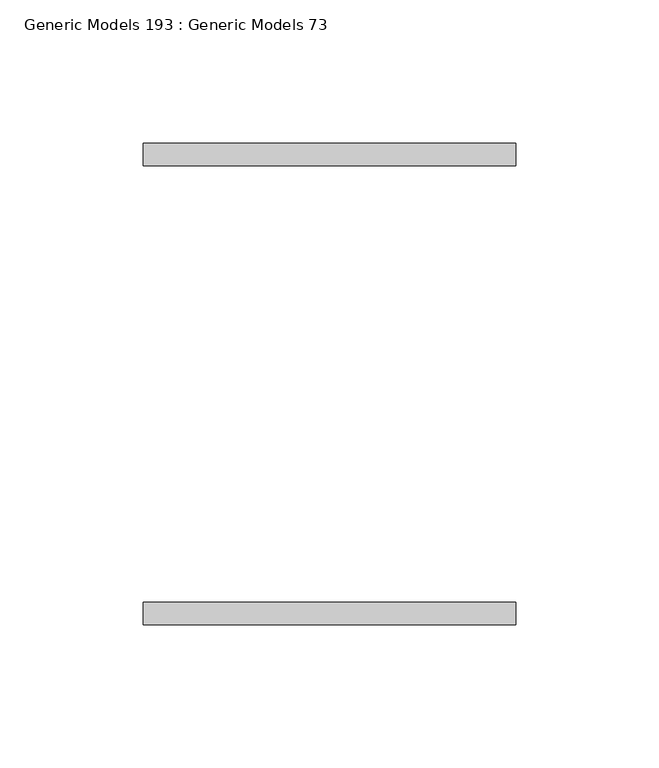
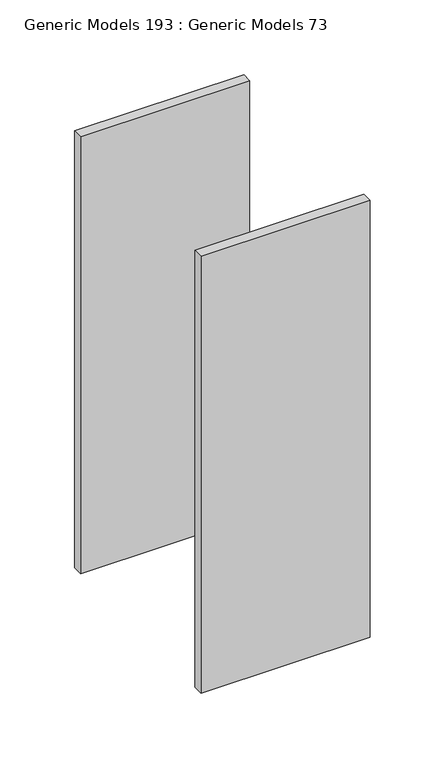
"""IFC4 building model written with IfcOpenShell, lengths in millimetres: proxy geometry, Generic Models 193 : Generic Models 73."""

import ifcopenshell
import ifcopenshell.guid

model = None  # the IFC model being written
_history = None  # IfcOwnerHistory: only IFC2X3 demands one
_inside = {}  # id of a spatial element -> (the spatial element, [elements in it])
_under = {}  # id of a project, library or spatial element -> (it, [spatial elements below it])
_declared = {}  # id of a project -> (the project, [libraries it declares])
_typed = {}  # id of a type object -> (the type object, [elements of that type])
_made_of = {}  # id of a material, layer set ... -> (it, [elements and type objects made of it])


def new_model(schema):
    """Start an empty IFC model of exactly this schema.

    Asked for "IFC4X3", IfcOpenShell would pick the latest addendum, in which some entities
    have other attributes; the version numbers below select the first issue.
    IFC2X3 requires an IfcOwnerHistory on every rooted entity: one is made here for all.
    """
    global model, _history
    if schema == "IFC4X3":
        model = ifcopenshell.file(schema_version=(4, 3, 0, 0))
    else:
        model = ifcopenshell.file(schema=schema)
    _inside.clear()
    _under.clear()
    _declared.clear()
    _typed.clear()
    _made_of.clear()
    _history = None
    if model.schema == "IFC2X3":
        org = make("IfcOrganization", Name="unknown")
        user = make(
            "IfcPersonAndOrganization",
            ThePerson=make("IfcPerson", FamilyName="unknown"),
            TheOrganization=org,
        )
        app = make(
            "IfcApplication",
            ApplicationDeveloper=org,
            Version="unknown",
            ApplicationFullName="unknown",
            ApplicationIdentifier="unknown",
        )
        _history = make(
            "IfcOwnerHistory",
            OwningUser=user,
            OwningApplication=app,
            ChangeAction="ADDED",
            CreationDate=0,
        )
    return model


def make(cls, **values):
    """One entity of the class cls with the attributes given. An attribute that is None is left unset."""
    return model.create_entity(
        cls, **{name: value for name, value in values.items() if value is not None}
    )


def rooted(cls, **values):
    """An entity with a GlobalId (a new one), such as an element, a storey or a relation."""
    return make(cls, GlobalId=ifcopenshell.guid.new(), OwnerHistory=_history, **values)


def si_unit(unit_type, name, prefix=None):
    """IfcSIUnit, for example si_unit("LENGTHUNIT", "METRE", prefix="MILLI")."""
    return make("IfcSIUnit", UnitType=unit_type, Prefix=prefix, Name=name)


def assignment(units):
    """IfcUnitAssignment: the units of a project."""
    return None if units is None else make("IfcUnitAssignment", Units=units)


def point(xyz):
    """IfcCartesianPoint."""
    return None if xyz is None else make("IfcCartesianPoint", Coordinates=xyz)


def direction(xyz):
    """IfcDirection."""
    return None if xyz is None else make("IfcDirection", DirectionRatios=xyz)


def frame(location, z_axis=None, x_axis=None):
    """IfcAxis2Placement3D, a coordinate frame: its origin and axes. An axis left out is left unset."""
    return make(
        "IfcAxis2Placement3D",
        Location=point(location),
        Axis=direction(z_axis),
        RefDirection=direction(x_axis),
    )


def origin():
    """The frame at (0, 0, 0) with its axes left unset."""
    return frame((0.0, 0.0, 0.0))


def place(relative_to, where):
    """IfcLocalPlacement: puts the frame where relative to a parent placement (None: the world)."""
    return make(
        "IfcLocalPlacement", PlacementRelTo=relative_to, RelativePlacement=where
    )


def context(
    kind, dimensions, precision=None, world=None, true_north=None, identifier=None
):
    """IfcGeometricRepresentationContext, for example the 3D "Model" context."""
    return make(
        "IfcGeometricRepresentationContext",
        ContextIdentifier=identifier,
        ContextType=kind,
        CoordinateSpaceDimension=dimensions,
        Precision=precision,
        WorldCoordinateSystem=world,
        TrueNorth=true_north,
    )


def project(units=None, contexts=None):
    """IfcProject with its units and contexts."""
    return rooted(
        "IfcProject",
        Name="project",
        RepresentationContexts=contexts,
        UnitsInContext=assignment(units),
    )


def spatial(cls, under=None, at=None, **own):
    """A site, building, storey or space (cls), placed at a placement, below another one or the project."""
    s = rooted(cls, ObjectPlacement=at, **own)
    if under is not None:
        _under.setdefault(under.id(), (under, []))[1].append(s)
    return s


def polyline(points):
    """IfcPolyline through the points."""
    return make("IfcPolyline", Points=[point(p) for p in points])


def outline(outer, holes=None, kind="AREA"):
    """IfcArbitraryClosedProfileDef: a profile drawn as a closed curve; with holes, ...WithVoids."""
    if holes is None:
        return make("IfcArbitraryClosedProfileDef", ProfileType=kind, OuterCurve=outer)
    return make(
        "IfcArbitraryProfileDefWithVoids",
        ProfileType=kind,
        OuterCurve=outer,
        InnerCurves=holes,
    )


def extrude(swept, where, along, depth):
    """IfcExtrudedAreaSolid: the profile swept, set in the frame where, extruded along a direction by depth."""
    return make(
        "IfcExtrudedAreaSolid",
        SweptArea=swept,
        Position=where,
        ExtrudedDirection=direction(along),
        Depth=depth,
    )


def shape(context_of_items, identifier, shape_type, items):
    """IfcShapeRepresentation: the items that make up one representation, for example the "Body"."""
    return make(
        "IfcShapeRepresentation",
        ContextOfItems=context_of_items,
        RepresentationIdentifier=identifier,
        RepresentationType=shape_type,
        Items=items,
    )


def source(mapping_origin, context_of_items, identifier, shape_type, items):
    """IfcRepresentationMap: a shape defined once, which mapped items show again and again."""
    return make(
        "IfcRepresentationMap",
        MappingOrigin=mapping_origin,
        MappedRepresentation=shape(context_of_items, identifier, shape_type, items),
    )


def transform(
    local_origin,
    x_axis=None,
    y_axis=None,
    z_axis=None,
    scale=None,
    scale2=None,
    scale3=None,
    uniform=True,
):
    """IfcCartesianTransformationOperator3D, or its non-uniform kind. x_axis, y_axis, z_axis: its Axis1, 2, 3."""
    if uniform:
        return make(
            "IfcCartesianTransformationOperator3D",
            Axis1=direction(x_axis),
            Axis2=direction(y_axis),
            LocalOrigin=point(local_origin),
            Scale=scale,
            Axis3=direction(z_axis),
        )
    return make(
        "IfcCartesianTransformationOperator3DnonUniform",
        Axis1=direction(x_axis),
        Axis2=direction(y_axis),
        LocalOrigin=point(local_origin),
        Scale=scale,
        Axis3=direction(z_axis),
        Scale2=scale2,
        Scale3=scale3,
    )


def mapped(mapping_source, mapping_target):
    """IfcMappedItem: shows the shape of a source again, moved by a transform."""
    return make(
        "IfcMappedItem", MappingSource=mapping_source, MappingTarget=mapping_target
    )


def made_of(thing, what):
    """Note that an element or type object is made of a material, layer set ...; save() writes the relation."""
    if what is not None:
        _made_of.setdefault(what.id(), (what, []))[1].append(thing)
    return thing


def element(
    cls,
    number,
    at=None,
    inside=None,
    cuts=None,
    type_object=None,
    material=None,
    context=None,
    identifier="Body",
    shape_type=None,
    held_by="IfcProductDefinitionShape",
    body=None,
    shapes=None,
    **own,
):
    """One element of the class cls, such as IfcWall. Its Tag is "e" and its number.

    at: its placement. inside: the storey or other place that contains it. cuts: it is an
    opening in that element (IfcRelVoidsElement). A single representation is given by context,
    identifier, shape_type and body (its items); several are given by shapes. held_by: the class
    of the entity that holds the representations. save() writes the other relations.
    """
    e = rooted(cls, Tag="e%d" % number, ObjectPlacement=at, **own)
    if body is not None:
        shapes = [shape(context, identifier, shape_type, body)]
    if shapes is not None:
        e.Representation = make(held_by, Representations=shapes)
    if inside is not None:
        _inside.setdefault(inside.id(), (inside, []))[1].append(e)
    if cuts is not None:
        rooted(
            "IfcRelVoidsElement", RelatingBuildingElement=cuts, RelatedOpeningElement=e
        )
    if type_object is not None:
        _typed.setdefault(type_object.id(), (type_object, []))[1].append(e)
    return made_of(e, material)


def aggregate(whole, parts):
    """IfcRelAggregates: a whole, such as a stair, and the parts it consists of."""
    return rooted("IfcRelAggregates", RelatingObject=whole, RelatedObjects=parts)


def save(model, path):
    """Write the relations noted so far, then the file.

    IfcRelAggregates (storeys below a building ...), IfcRelContainedInSpatialStructure (elements
    in a storey), IfcRelDefinesByType, IfcRelAssociatesMaterial and IfcRelDeclares: one each for
    every whole, place, type object, material and project.
    """
    for whole, parts in _under.values():
        aggregate(whole, parts)
    for where, things in _inside.values():
        rooted(
            "IfcRelContainedInSpatialStructure",
            RelatedElements=things,
            RelatingStructure=where,
        )
    for kind, things in _typed.values():
        rooted("IfcRelDefinesByType", RelatedObjects=things, RelatingType=kind)
    for what, things in _made_of.values():
        rooted("IfcRelAssociatesMaterial", RelatedObjects=things, RelatingMaterial=what)
    for by, libraries in _declared.values():
        rooted("IfcRelDeclares", RelatingContext=by, RelatedDefinitions=libraries)
    model.write(path)


def generic_models_193_generic_models_73_41cc18d0(model_context):
    return source(origin(), model_context, "Body", "SweptSolid", [
        extrude(outline(polyline([(32040.4971032, 36491.5582942), (32040.4971032, 36483.6207942), (31910.3221032, 36483.6207942), (31910.3221032, 36491.5582942), (32040.4971032, 36491.5582942)])), frame((0.0, 0.0, 268393.8625), z_axis=(0.0, 0.0, 1.0), x_axis=(1.0, 0.0, 0.0)), (0.0, 0.0, 1.0), 355.6),
        extrude(outline(polyline([(32040.4971032, 36331.2207942), (32040.4971032, 36323.2832942), (31910.3221032, 36323.2832942), (31910.3221032, 36331.2207942), (32040.4971032, 36331.2207942)])), frame((0.0, 0.0, 268393.8625), z_axis=(0.0, 0.0, 1.0), x_axis=(1.0, 0.0, 0.0)), (0.0, 0.0, 1.0), 355.6),
    ])


if __name__ == "__main__":
    model = new_model("IFC4")
    model_context = context("Model", 3, world=origin())
    ifc_project = project(units=[si_unit("LENGTHUNIT", "METRE", prefix="MILLI")], contexts=[model_context])
    site = spatial("IfcSite", under=ifc_project)
    building = spatial("IfcBuilding", under=site)
    placement = place(None, origin())
    generic_models_193_generic_models_73_shape = generic_models_193_generic_models_73_41cc18d0(model_context)
    element("IfcBuildingElementProxy", 1, Name="Generic Models 193 : Generic Models 73", ObjectType="Generic Models 193 : Generic Models 73", at=placement, inside=building, context=model_context, shape_type="MappedRepresentation", body=[
        mapped(generic_models_193_generic_models_73_shape, transform((0.0, 0.0, 0.0), x_axis=(1.0, 0.0, 0.0), y_axis=(0.0, 1.0, 0.0), z_axis=(0.0, 0.0, 1.0))),
    ])
    save(model, "model.ifc")

# Revit data of these elements
# Element 1 (IfcBuildingElementProxy, "Generic Models 193 : Generic Models 73")
#   Materials on its faces: "5/16 x 9 x 1'-2\" SIDE PLATES  CAP\nW/ 2 3/4\"DIA. THRU BOLTS"
# Materials
#   "5/16 x 9 x 1'-2\" SIDE PLATES  CAP\nW/ 2 3/4\"DIA. THRU BOLTS": class "Metal", colour RGB 199 199 199, transparency 0, Description = "Carbon steel", Cost = 0
